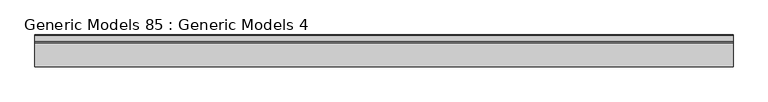
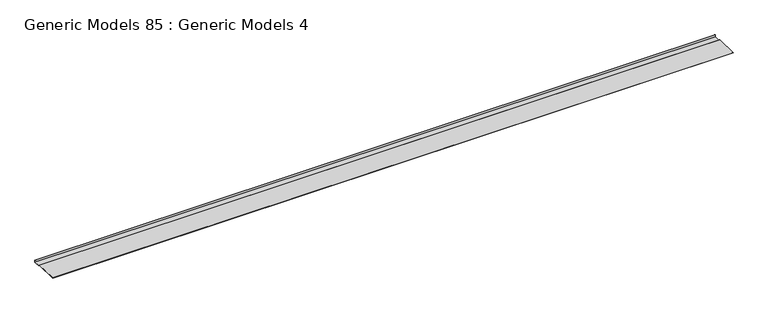
"""IFC4 building model written with IfcOpenShell, lengths in millimetres: proxy geometry, Generic Models 85 : Generic Models 4."""

from ifc_helpers import new_model, si_unit, frame, origin, place, context, project, spatial, polyline, outline, extrude, source, transform, mapped, element, save


def generic_models_85_generic_models_4_10e6c794(model_context):
    return source(origin(), model_context, "Body", "SweptSolid", [
        extrude(outline(polyline([(-24488.4131016, 126324.2668254), (-24477.3282619, 126311.40973), (-24420.0761295, 126310.4590779), (-24420.0761295, 126328.6067839), (-24419.1216671, 126328.6067839), (-24419.1216671, 126309.5567839), (-24477.9737102, 126310.546932), (-24488.9610286, 126323.4758345), (-24701.2399614, 126327.8983122), (-24701.2234285, 126328.6918901), (-24488.4131016, 126324.2668254)])), frame((2196.9263704, 0.0, 0.0), z_axis=(1.0, 0.0, 0.0), x_axis=(0.0, 1.0, 0.0)), (0.0, 0.0, 1.0), 6212.156498),
    ])


if __name__ == "__main__":
    model = new_model("IFC4")
    model_context = context("Model", 3, world=origin())
    ifc_project = project(units=[si_unit("LENGTHUNIT", "METRE", prefix="MILLI")], contexts=[model_context])
    site = spatial("IfcSite", under=ifc_project)
    building = spatial("IfcBuilding", under=site)
    placement = place(None, origin())
    generic_models_85_generic_models_4_shape = generic_models_85_generic_models_4_10e6c794(model_context)
    element("IfcBuildingElementProxy", 1, Name="Generic Models 85 : Generic Models 4", ObjectType="Generic Models 85 : Generic Models 4", at=placement, inside=building, context=model_context, shape_type="MappedRepresentation", body=[
        mapped(generic_models_85_generic_models_4_shape, transform((0.0, 0.0, 0.0), x_axis=(1.0, 0.0, 0.0), y_axis=(0.0, 1.0, 0.0), z_axis=(0.0, 0.0, 1.0))),
    ])
    save(model, "model.ifc")

# Revit data of these elements
# Element 1 (IfcBuildingElementProxy, "Generic Models 85 : Generic Models 4")
#   Materials on its faces: "_HYDROSTOP LIQUID MEMBRANE - FOLLOW MANU. RECOMMENDED INSTALLATION DETAILS"
# Materials
#   "_HYDROSTOP LIQUID MEMBRANE - FOLLOW MANU. RECOMMENDED INSTALLATION DETAILS": class "Generic", colour RGB 156 184 169, transparency 0, Cost = 0
